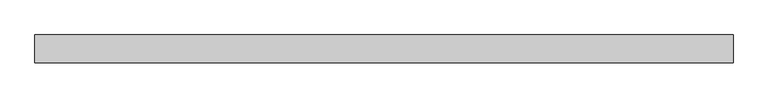
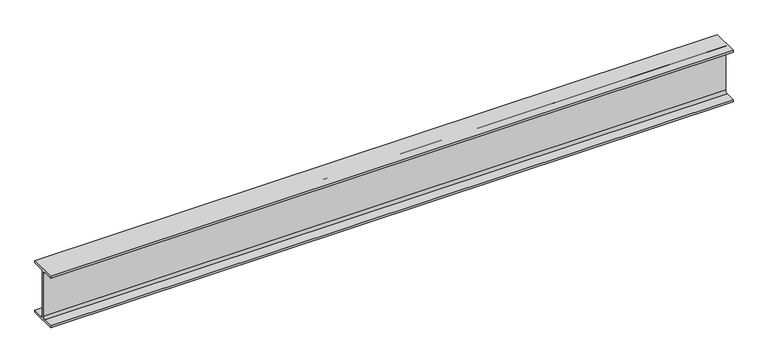
"""IFC4 building model written with IfcOpenShell, lengths in millimetres: beam geometry, 0912_Steel Framing_H-KSD3502 : H_SB_ASB_H-250x125x6x9."""

from ifc_helpers import new_model, si_unit, point, frame, frame_2d, origin, place, context, project, spatial, polyline, circle_curve, trimmed, segment, composite_curve, outline, extrude, source, transform, mapped, element, save


def beam_d4d7e5cf(model_context):
    return source(origin(), model_context, "Body", "SweptSolid", [
        extrude(outline(composite_curve([segment(polyline([(62.5, -116.0), (62.5, -125.0), (-62.5, -125.0), (-62.5, -116.0), (-15.0, -116.0)]), True, "CONTINUOUS"), segment(trimmed(circle_curve(frame_2d((-15.0, -104.0)), 12.0), [point((-15.0, -116.0))], [point((-3.0, -104.0))], True, "CARTESIAN"), True, "CONTINUOUS"), segment(polyline([(-3.0, -104.0), (-3.0, 104.0)]), True, "CONTINUOUS"), segment(trimmed(circle_curve(frame_2d((-15.0, 104.0)), 12.0), [point((-3.0, 104.0))], [point((-15.0, 116.0))], True, "CARTESIAN"), True, "CONTINUOUS"), segment(polyline([(-15.0, 116.0), (-62.5, 116.0), (-62.5, 125.0), (62.5, 125.0), (62.5, 116.0), (15.0, 116.0)]), True, "CONTINUOUS"), segment(trimmed(circle_curve(frame_2d((15.0, 104.0)), 12.0), [point((15.0, 116.0))], [point((3.0, 104.0))], True, "CARTESIAN"), True, "CONTINUOUS"), segment(polyline([(3.0, 104.0), (3.0, -104.0)]), True, "CONTINUOUS"), segment(trimmed(circle_curve(frame_2d((15.0, -104.0)), 12.0), [point((3.0, -104.0))], [point((15.0, -116.0))], True, "CARTESIAN"), True, "CONTINUOUS"), segment(polyline([(15.0, -116.0), (62.5, -116.0)]), True, "CONTINUOUS")], self_intersect=False)), frame((-1494.4889476, 0.0, 0.0), z_axis=(1.0, 0.0, 0.0), x_axis=(0.0, 1.0, 0.0)), (0.0, 0.0, 1.0), 3149.288991),
    ])


if __name__ == "__main__":
    model = new_model("IFC4")
    model_context = context("Model", 3, world=origin())
    ifc_project = project(units=[si_unit("LENGTHUNIT", "METRE", prefix="MILLI")], contexts=[model_context])
    site = spatial("IfcSite", under=ifc_project)
    building = spatial("IfcBuilding", under=site)
    placement = place(None, origin())
    beam_shape = beam_d4d7e5cf(model_context)
    element("IfcBeam", 1, ObjectType="0912_Steel Framing_H-KSD3502 : H_SB_ASB_H-250x125x6x9", at=placement, inside=building, context=model_context, shape_type="MappedRepresentation", body=[
        mapped(beam_shape, transform((0.0, 0.0, 0.0), x_axis=(1.0, 0.0, 0.0), y_axis=(0.0, 1.0, 0.0), z_axis=(0.0, 0.0, 1.0))),
    ])
    save(model, "model.ifc")

# Revit data of these elements
# Type "0912_Steel Framing_H-KSD3502 : H_SB_ASB_H-250x125x6x9"
#   H_WM Code_1 = "S01AA003-00001 | Main Steel Structure Fabrication Work | Shelter/Building | Light Steel - Standard (30KG/M>Weight) | Material: (   )"
#   H_WM Code_2 = "S03AA029-00001 | Main Steel Structure Erection Work | Shelter/Building | Light Steel (30KG/M>Weight) | Material: (   )"
#   H_WM Code_3 = "S01AA010-00001 | Main Steel Structure Fabrication Work | Shelter/Building | Steel Painting/Coating | for Non-Fireproofed Steel Surface, Surface Preparation, Primer, Second & Final Coat | Material: (   )"
#   H_Q'ty Cal Type Tag = "SB-Q2"
#   Width = 12.5 cm
#   Web Thickness = 0.6 cm
#   Web Fillet = 1.2 cm
#   Warping Constant = 42539.8 cm⁶
#   W = 0
#   Torsional Moment of Inertia = 7.8102 cm⁴
#   Section Area = 37.66 cm²
#   Plastic Modulus weak axis = 73.1 cm³
#   Plastic Modulus strong axis = 366.0 cm³
#   Perimeter = 0.97 m²/m
#   Nominal Weight = 29.60 kgf/m
#   Moment of Inertia weak axis = 294.00 cm⁴
#   Moment of Inertia strong axis = 4050.00 cm⁴
#   Height = 25.0 cm
#   Flange Thickness = 0.9 cm
#   Elastic Modulus weak axis = 47.0 cm³
#   Elastic Modulus strong axis = 324.0 cm³
#   Centroid Vertical = 12.5 cm
#   Centroid Horizontal = 6.25 cm
#   Ix = 40500000
#   Length [instance default] = 1.5240 m
#   Zx = 366000
#   b = 0.1250 m
#   h = 0.2500 m
#   r = 0.0120 m
#   s = 0.0060 m
#   t = 0.0090 m
#   A = 0.003766 m²
#   Structural Material [instance default] = Steel, 45-345
#   Assembly Code = ""
# Element 1 (IfcBeam, "0912_Steel Framing_H-KSD3502 : H_SB_ASB_H-250x125x6x9")
#   Structural Material = none
# Materials
#   "Steel, 45-345": class "Metal", colour RGB 189 187 185, transparency 0, Description = "Steel 345 MPa", Cost = 0
